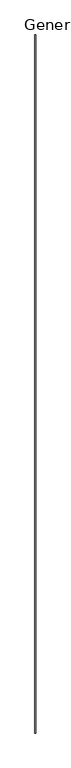
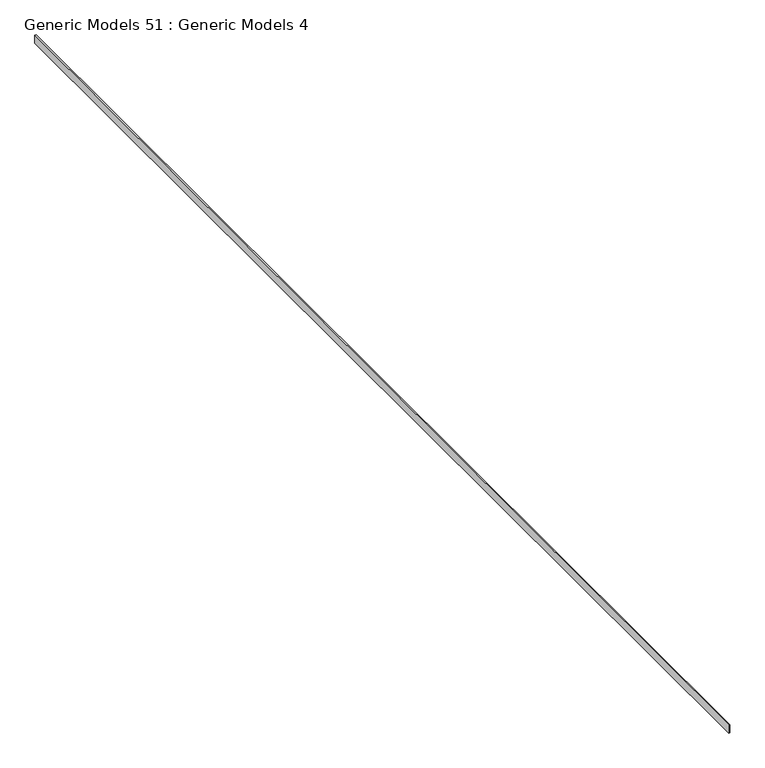
"""IFC4 building model written with IfcOpenShell, lengths in millimetres: proxy geometry, Generic Models 51 : Generic Models 4."""

import ifcopenshell
import ifcopenshell.guid

model = None  # the IFC model being written
_history = None  # IfcOwnerHistory: only IFC2X3 demands one
_inside = {}  # id of a spatial element -> (the spatial element, [elements in it])
_under = {}  # id of a project, library or spatial element -> (it, [spatial elements below it])
_declared = {}  # id of a project -> (the project, [libraries it declares])
_typed = {}  # id of a type object -> (the type object, [elements of that type])
_made_of = {}  # id of a material, layer set ... -> (it, [elements and type objects made of it])


def new_model(schema):
    """Start an empty IFC model of exactly this schema.

    Asked for "IFC4X3", IfcOpenShell would pick the latest addendum, in which some entities
    have other attributes; the version numbers below select the first issue.
    IFC2X3 requires an IfcOwnerHistory on every rooted entity: one is made here for all.
    """
    global model, _history
    if schema == "IFC4X3":
        model = ifcopenshell.file(schema_version=(4, 3, 0, 0))
    else:
        model = ifcopenshell.file(schema=schema)
    _inside.clear()
    _under.clear()
    _declared.clear()
    _typed.clear()
    _made_of.clear()
    _history = None
    if model.schema == "IFC2X3":
        org = make("IfcOrganization", Name="unknown")
        user = make(
            "IfcPersonAndOrganization",
            ThePerson=make("IfcPerson", FamilyName="unknown"),
            TheOrganization=org,
        )
        app = make(
            "IfcApplication",
            ApplicationDeveloper=org,
            Version="unknown",
            ApplicationFullName="unknown",
            ApplicationIdentifier="unknown",
        )
        _history = make(
            "IfcOwnerHistory",
            OwningUser=user,
            OwningApplication=app,
            ChangeAction="ADDED",
            CreationDate=0,
        )
    return model


def make(cls, **values):
    """One entity of the class cls with the attributes given. An attribute that is None is left unset."""
    return model.create_entity(
        cls, **{name: value for name, value in values.items() if value is not None}
    )


def rooted(cls, **values):
    """An entity with a GlobalId (a new one), such as an element, a storey or a relation."""
    return make(cls, GlobalId=ifcopenshell.guid.new(), OwnerHistory=_history, **values)


def si_unit(unit_type, name, prefix=None):
    """IfcSIUnit, for example si_unit("LENGTHUNIT", "METRE", prefix="MILLI")."""
    return make("IfcSIUnit", UnitType=unit_type, Prefix=prefix, Name=name)


def assignment(units):
    """IfcUnitAssignment: the units of a project."""
    return None if units is None else make("IfcUnitAssignment", Units=units)


def point(xyz):
    """IfcCartesianPoint."""
    return None if xyz is None else make("IfcCartesianPoint", Coordinates=xyz)


def direction(xyz):
    """IfcDirection."""
    return None if xyz is None else make("IfcDirection", DirectionRatios=xyz)


def frame(location, z_axis=None, x_axis=None):
    """IfcAxis2Placement3D, a coordinate frame: its origin and axes. An axis left out is left unset."""
    return make(
        "IfcAxis2Placement3D",
        Location=point(location),
        Axis=direction(z_axis),
        RefDirection=direction(x_axis),
    )


def origin():
    """The frame at (0, 0, 0) with its axes left unset."""
    return frame((0.0, 0.0, 0.0))


def place(relative_to, where):
    """IfcLocalPlacement: puts the frame where relative to a parent placement (None: the world)."""
    return make(
        "IfcLocalPlacement", PlacementRelTo=relative_to, RelativePlacement=where
    )


def context(
    kind, dimensions, precision=None, world=None, true_north=None, identifier=None
):
    """IfcGeometricRepresentationContext, for example the 3D "Model" context."""
    return make(
        "IfcGeometricRepresentationContext",
        ContextIdentifier=identifier,
        ContextType=kind,
        CoordinateSpaceDimension=dimensions,
        Precision=precision,
        WorldCoordinateSystem=world,
        TrueNorth=true_north,
    )


def project(units=None, contexts=None):
    """IfcProject with its units and contexts."""
    return rooted(
        "IfcProject",
        Name="project",
        RepresentationContexts=contexts,
        UnitsInContext=assignment(units),
    )


def spatial(cls, under=None, at=None, **own):
    """A site, building, storey or space (cls), placed at a placement, below another one or the project."""
    s = rooted(cls, ObjectPlacement=at, **own)
    if under is not None:
        _under.setdefault(under.id(), (under, []))[1].append(s)
    return s


def polyline(points):
    """IfcPolyline through the points."""
    return make("IfcPolyline", Points=[point(p) for p in points])


def outline(outer, holes=None, kind="AREA"):
    """IfcArbitraryClosedProfileDef: a profile drawn as a closed curve; with holes, ...WithVoids."""
    if holes is None:
        return make("IfcArbitraryClosedProfileDef", ProfileType=kind, OuterCurve=outer)
    return make(
        "IfcArbitraryProfileDefWithVoids",
        ProfileType=kind,
        OuterCurve=outer,
        InnerCurves=holes,
    )


def extrude(swept, where, along, depth):
    """IfcExtrudedAreaSolid: the profile swept, set in the frame where, extruded along a direction by depth."""
    return make(
        "IfcExtrudedAreaSolid",
        SweptArea=swept,
        Position=where,
        ExtrudedDirection=direction(along),
        Depth=depth,
    )


def shape(context_of_items, identifier, shape_type, items):
    """IfcShapeRepresentation: the items that make up one representation, for example the "Body"."""
    return make(
        "IfcShapeRepresentation",
        ContextOfItems=context_of_items,
        RepresentationIdentifier=identifier,
        RepresentationType=shape_type,
        Items=items,
    )


def source(mapping_origin, context_of_items, identifier, shape_type, items):
    """IfcRepresentationMap: a shape defined once, which mapped items show again and again."""
    return make(
        "IfcRepresentationMap",
        MappingOrigin=mapping_origin,
        MappedRepresentation=shape(context_of_items, identifier, shape_type, items),
    )


def transform(
    local_origin,
    x_axis=None,
    y_axis=None,
    z_axis=None,
    scale=None,
    scale2=None,
    scale3=None,
    uniform=True,
):
    """IfcCartesianTransformationOperator3D, or its non-uniform kind. x_axis, y_axis, z_axis: its Axis1, 2, 3."""
    if uniform:
        return make(
            "IfcCartesianTransformationOperator3D",
            Axis1=direction(x_axis),
            Axis2=direction(y_axis),
            LocalOrigin=point(local_origin),
            Scale=scale,
            Axis3=direction(z_axis),
        )
    return make(
        "IfcCartesianTransformationOperator3DnonUniform",
        Axis1=direction(x_axis),
        Axis2=direction(y_axis),
        LocalOrigin=point(local_origin),
        Scale=scale,
        Axis3=direction(z_axis),
        Scale2=scale2,
        Scale3=scale3,
    )


def mapped(mapping_source, mapping_target):
    """IfcMappedItem: shows the shape of a source again, moved by a transform."""
    return make(
        "IfcMappedItem", MappingSource=mapping_source, MappingTarget=mapping_target
    )


def made_of(thing, what):
    """Note that an element or type object is made of a material, layer set ...; save() writes the relation."""
    if what is not None:
        _made_of.setdefault(what.id(), (what, []))[1].append(thing)
    return thing


def element(
    cls,
    number,
    at=None,
    inside=None,
    cuts=None,
    type_object=None,
    material=None,
    context=None,
    identifier="Body",
    shape_type=None,
    held_by="IfcProductDefinitionShape",
    body=None,
    shapes=None,
    **own,
):
    """One element of the class cls, such as IfcWall. Its Tag is "e" and its number.

    at: its placement. inside: the storey or other place that contains it. cuts: it is an
    opening in that element (IfcRelVoidsElement). A single representation is given by context,
    identifier, shape_type and body (its items); several are given by shapes. held_by: the class
    of the entity that holds the representations. save() writes the other relations.
    """
    e = rooted(cls, Tag="e%d" % number, ObjectPlacement=at, **own)
    if body is not None:
        shapes = [shape(context, identifier, shape_type, body)]
    if shapes is not None:
        e.Representation = make(held_by, Representations=shapes)
    if inside is not None:
        _inside.setdefault(inside.id(), (inside, []))[1].append(e)
    if cuts is not None:
        rooted(
            "IfcRelVoidsElement", RelatingBuildingElement=cuts, RelatedOpeningElement=e
        )
    if type_object is not None:
        _typed.setdefault(type_object.id(), (type_object, []))[1].append(e)
    return made_of(e, material)


def aggregate(whole, parts):
    """IfcRelAggregates: a whole, such as a stair, and the parts it consists of."""
    return rooted("IfcRelAggregates", RelatingObject=whole, RelatedObjects=parts)


def save(model, path):
    """Write the relations noted so far, then the file.

    IfcRelAggregates (storeys below a building ...), IfcRelContainedInSpatialStructure (elements
    in a storey), IfcRelDefinesByType, IfcRelAssociatesMaterial and IfcRelDeclares: one each for
    every whole, place, type object, material and project.
    """
    for whole, parts in _under.values():
        aggregate(whole, parts)
    for where, things in _inside.values():
        rooted(
            "IfcRelContainedInSpatialStructure",
            RelatedElements=things,
            RelatingStructure=where,
        )
    for kind, things in _typed.values():
        rooted("IfcRelDefinesByType", RelatedObjects=things, RelatingType=kind)
    for what, things in _made_of.values():
        rooted("IfcRelAssociatesMaterial", RelatedObjects=things, RelatingMaterial=what)
    for by, libraries in _declared.values():
        rooted("IfcRelDeclares", RelatingContext=by, RelatedDefinitions=libraries)
    model.write(path)


def generic_models_51_generic_models_4_21c653b1(model_context):
    return source(origin(), model_context, "Body", "SweptSolid", [
        extrude(outline(polyline([(8346.0514146, -6864.9230338), (8327.0014146, -6864.9230338), (8327.0014146, 11778.6769662), (8346.0514146, 11778.6769662), (8346.0514146, -6864.9230338)])), frame((0.0, 0.0, 126809.341198), z_axis=(0.0, 0.0, 1.0), x_axis=(1.0, 0.0, 0.0)), (0.0, 0.0, 1.0), 132.6610303),
    ])


if __name__ == "__main__":
    model = new_model("IFC4")
    model_context = context("Model", 3, world=origin())
    ifc_project = project(units=[si_unit("LENGTHUNIT", "METRE", prefix="MILLI")], contexts=[model_context])
    site = spatial("IfcSite", under=ifc_project)
    building = spatial("IfcBuilding", under=site)
    placement = place(None, origin())
    generic_models_51_generic_models_4_shape = generic_models_51_generic_models_4_21c653b1(model_context)
    element("IfcBuildingElementProxy", 1, Name="Generic Models 51 : Generic Models 4", ObjectType="Generic Models 51 : Generic Models 4", at=placement, inside=building, context=model_context, shape_type="MappedRepresentation", body=[
        mapped(generic_models_51_generic_models_4_shape, transform((0.0, 0.0, 0.0), x_axis=(1.0, 0.0, 0.0), y_axis=(0.0, 1.0, 0.0), z_axis=(0.0, 0.0, 1.0))),
    ])
    save(model, "model.ifc")

# Revit data of these elements
# Element 1 (IfcBuildingElementProxy, "Generic Models 51 : Generic Models 4")
#   Materials on its faces: "_CDX PLYWOOD - SEE STRUCT DWGs"
# Materials
#   "_CDX PLYWOOD - SEE STRUCT DWGs": class "Generic", colour RGB 98 75 74, transparency 0, Cost = 0
